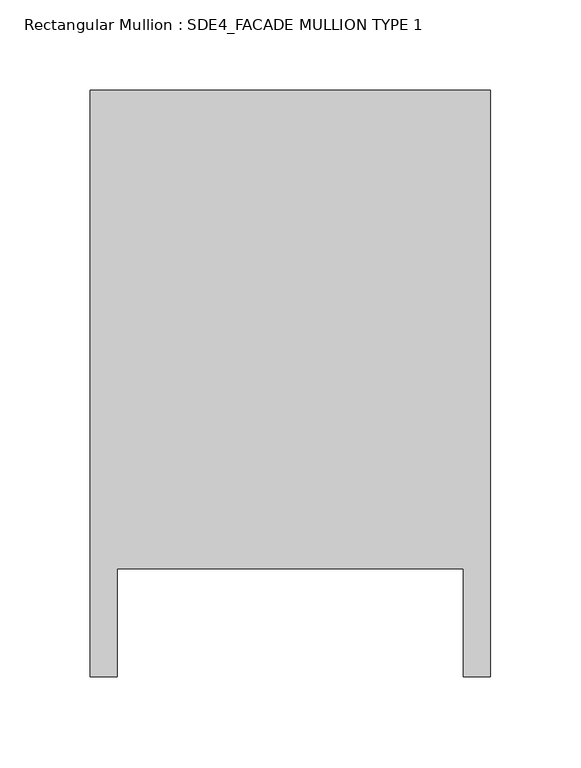
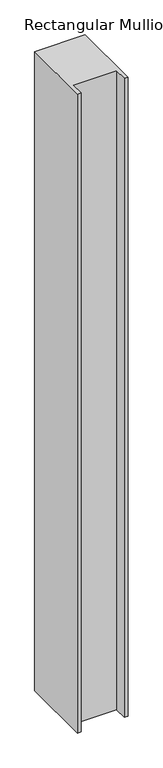
"""IFC4 building model written with IfcOpenShell, lengths in millimetres: member geometry, Rectangular Mullion : SDE4_FACADE MULLION TYPE 1."""

from ifc_helpers import new_model, si_unit, frame, origin, place, context, project, spatial, polyline, outline, extrude, source, transform, mapped, element, save


def rectangular_mullion_sde4_facade_mullion_type_1_f7d40089(model_context):
    return source(origin(), model_context, "Body", "SweptSolid", [
        extrude(outline(polyline([(111.0, 132.5), (111.0, -192.5), (96.0, -192.5), (96.0, -132.5), (-96.0, -132.5), (-96.0, -192.5), (-111.0, -192.5), (-111.0, 132.5), (111.0, 132.5)])), frame((0.0, 0.0, -2970.0), z_axis=(0.0, 0.0, 1.0), x_axis=(1.0, 0.0, 0.0)), (0.0, 0.0, 1.0), 2970.0),
    ])


if __name__ == "__main__":
    model = new_model("IFC4")
    model_context = context("Model", 3, world=origin())
    ifc_project = project(units=[si_unit("LENGTHUNIT", "METRE", prefix="MILLI")], contexts=[model_context])
    site = spatial("IfcSite", under=ifc_project)
    building = spatial("IfcBuilding", under=site)
    placement = place(None, origin())
    rectangular_mullion_sde4_facade_mullion_type_1_shape = rectangular_mullion_sde4_facade_mullion_type_1_f7d40089(model_context)
    element("IfcMember", 1, ObjectType="Rectangular Mullion : SDE4_FACADE MULLION TYPE 1", at=placement, inside=building, context=model_context, shape_type="MappedRepresentation", body=[
        mapped(rectangular_mullion_sde4_facade_mullion_type_1_shape, transform((0.0, 0.0, 0.0), x_axis=(1.0, 0.0, 0.0), y_axis=(0.0, 1.0, 0.0), z_axis=(0.0, 0.0, 1.0))),
    ])
    save(model, "model.ifc")

# Revit data of these elements
# Type "Rectangular Mullion : SDE4_FACADE MULLION TYPE 1"
#   built-in parameter 1007322 = 0.869423 (stored number, unit not read)
#   built-in parameter 1007321 = 0.364173 (stored number, unit not read)
#   built-in parameter 1007320 = 0.364173 (stored number, unit not read)
